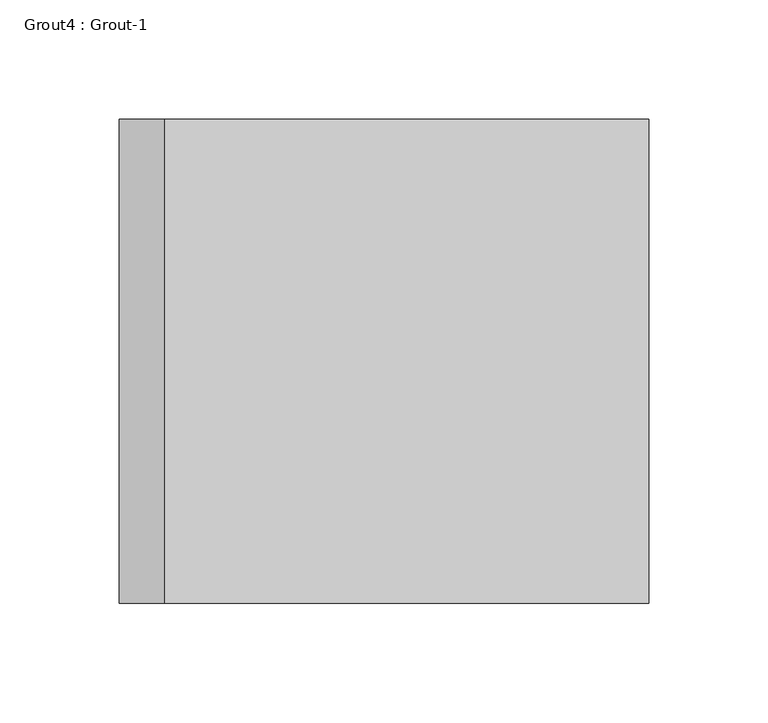
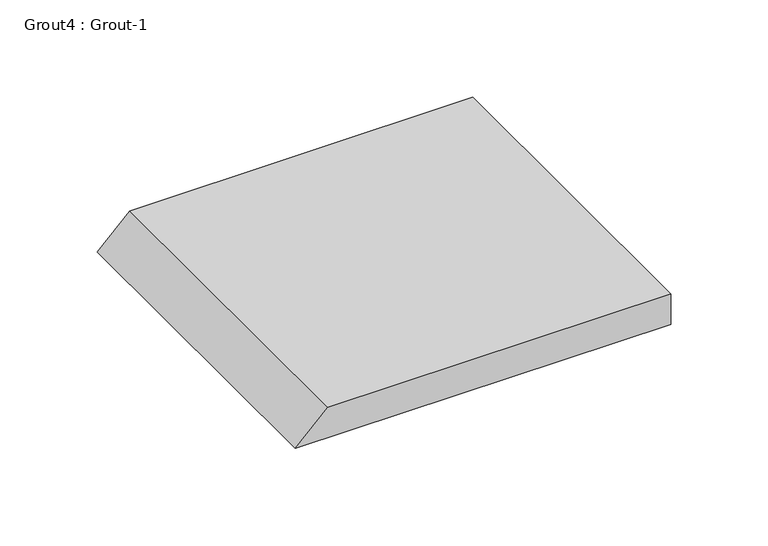
"""IFC4 building model written with IfcOpenShell, lengths in millimetres: proxy geometry, Grout4 : Grout-1."""

from ifc_helpers import new_model, si_unit, frame, origin, place, context, project, spatial, polyline, outline, extrude, source, transform, mapped, element, save


def grout4_grout_1_4b3d9b04(model_context):
    return source(origin(), model_context, "Body", "SweptSolid", [
        extrude(outline(polyline([(19.05, 590115.4434739), (0.0, 590096.3934739), (0.0, 590318.6434739), (19.05, 590318.6434739), (19.05, 590115.4434739)])), frame((0.0, -532982.2413841, 0.0), z_axis=(0.0, 1.0, 0.0), x_axis=(0.0, 0.0, 1.0)), (0.0, 0.0, 1.0), 203.2),
    ])


if __name__ == "__main__":
    model = new_model("IFC4")
    model_context = context("Model", 3, world=origin())
    ifc_project = project(units=[si_unit("LENGTHUNIT", "METRE", prefix="MILLI")], contexts=[model_context])
    site = spatial("IfcSite", under=ifc_project)
    building = spatial("IfcBuilding", under=site)
    placement = place(None, origin())
    grout4_grout_1_shape = grout4_grout_1_4b3d9b04(model_context)
    element("IfcBuildingElementProxy", 1, Name="Grout4 : Grout-1", ObjectType="Grout4 : Grout-1", at=placement, inside=building, context=model_context, shape_type="MappedRepresentation", body=[
        mapped(grout4_grout_1_shape, transform((0.0, 0.0, 0.0), x_axis=(1.0, 0.0, 0.0), y_axis=(0.0, 1.0, 0.0), z_axis=(0.0, 0.0, 1.0))),
    ])
    save(model, "model.ifc")

# Revit data of these elements
# Element 1 (IfcBuildingElementProxy, "Grout4 : Grout-1")
#   Materials on its faces: "3/4\" NON SHRINK GROUT"
# Materials
#   "3/4\" NON SHRINK GROUT": class "Generic", colour RGB 145 145 143, transparency 0, Cost = 0
